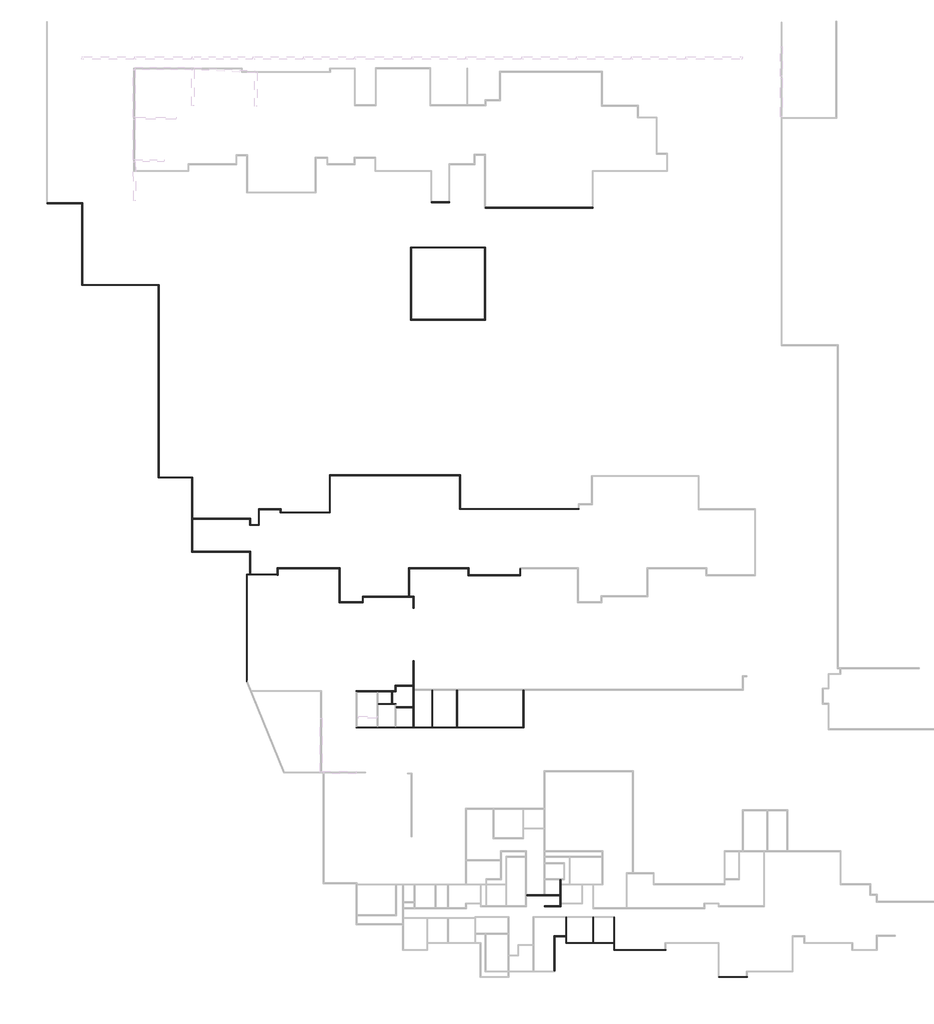
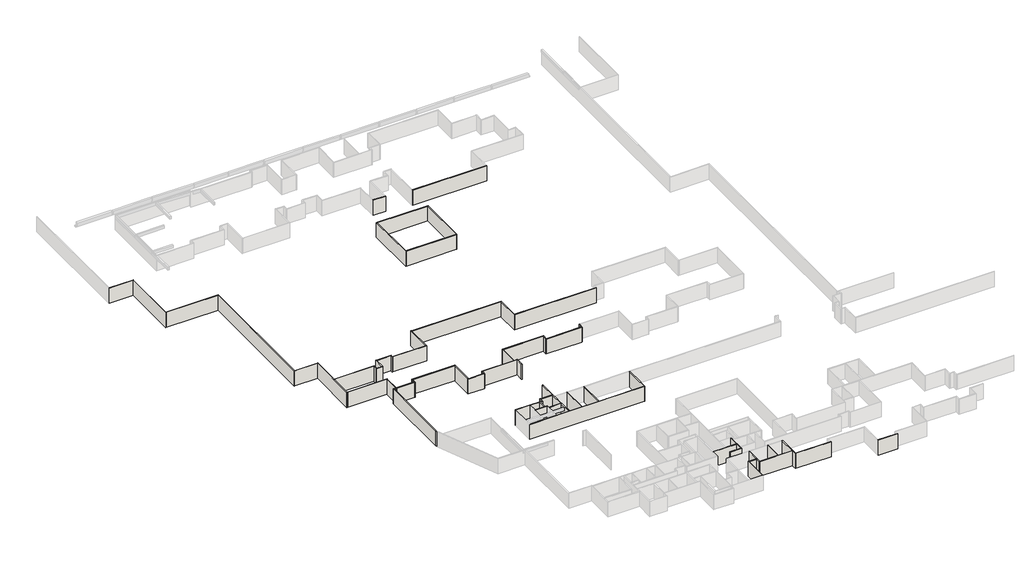
# One storey, part 2 of 8: 63 walls.
"""IFC4 building model written with IfcOpenShell, lengths in millimetres."""

from ifc_helpers import new_model, si_unit, origin, origin_with_axes, place, context, project, spatial, polyline, outline, extrude, faceted_brep, element, save

model = new_model("IFC4")

# Units and contexts
model_context = context("Model", 3, world=origin())
ifc_project = project(units=[si_unit("LENGTHUNIT", "METRE", prefix="MILLI")], contexts=[model_context])

# Site, building, storey
site = spatial("IfcSite", under=ifc_project)
building = spatial("IfcBuilding", under=site)
storey = spatial("IfcBuildingStorey", under=building, Name="户型图", Elevation=0.0)

# Walls
placement = place(None, origin())
element("IfcWall", 1, ObjectType="所有墙体", at=placement, inside=storey, context=model_context, shape_type="Brep", body=[
    faceted_brep([(57170.338145, 126907.0451941, 0.0), (62113.8430954, 126907.0451941, 0.0), (62113.8430954, 126907.0451941, 3300.0), (57170.338145, 126907.0451941, 3300.0), (57170.338145, 127027.0451941, 0.0), (57170.338145, 127027.0451941, 3300.0), (62108.8476291, 127027.0451941, 3300.0), (62113.8430954, 127027.0451941, 3300.0), (62113.8430954, 127027.0451941, 0.0)], [[[0, 1, 2, 3]], [[4, 5, 6, 7, 8]], [[1, 0, 4, 8]], [[3, 2, 7, 6, 5]], [[2, 1, 8, 7]], [[0, 3, 5, 4]]]),
])
element("IfcWall", 2, ObjectType="所有墙体", at=placement, inside=storey, context=model_context, shape_type="Brep", body=[
    faceted_brep([(62113.8430954, 127027.0451941, 0.0), (62113.8430954, 126907.0451941, 0.0), (62113.8430954, 115127.0451941, 0.0), (62113.8430954, 115127.0451941, 3300.0), (62113.8430954, 126907.0451941, 3300.0), (62113.8430954, 127027.0451941, 3300.0), (62233.8430954, 127027.0451941, 0.0), (62233.8430954, 127027.0451941, 2700.0), (62233.8430954, 127027.0451941, 3300.0), (62233.8430954, 126967.1449171, 3300.0), (62233.8430954, 115247.0451941, 3300.0), (62233.8430954, 115127.0451941, 3300.0), (62233.8430954, 115127.0451941, 0.0), (62233.8430954, 115247.0451941, 0.0)], [[[0, 1, 2, 3, 4, 5]], [[6, 7, 8, 9, 10, 11, 12, 13]], [[2, 1, 0, 6, 13, 12]], [[5, 4, 3, 11, 10, 9, 8]], [[0, 5, 8, 7, 6]], [[3, 2, 12, 11]]]),
])
element("IfcWall", 3, ObjectType="所有墙体", at=placement, inside=storey, context=model_context, shape_type="Brep", body=[
    faceted_brep([(62233.8430954, 115127.0451941, 0.0), (73113.8430954, 115127.0451941, 0.0), (73233.8430954, 115127.0451941, 0.0), (73233.8430954, 115127.0451941, 3300.0), (73113.8430954, 115127.0451941, 3300.0), (62233.8430954, 115127.0451941, 3300.0), (62233.8430954, 115247.0451941, 0.0), (62233.8430954, 115247.0451941, 3300.0), (73233.8430954, 115247.0451941, 3300.0), (73233.8430954, 115247.0451941, 0.0)], [[[0, 1, 2, 3, 4, 5]], [[6, 7, 8, 9]], [[2, 1, 0, 6, 9]], [[5, 4, 3, 8, 7]], [[0, 5, 7, 6]], [[3, 2, 9, 8]]]),
])
element("IfcWall", 4, ObjectType="所有墙体", at=placement, inside=storey, context=model_context, shape_type="Brep", body=[
    faceted_brep([(73113.8430954, 115127.0451941, 0.0), (73113.8430954, 87427.0451941, 0.0), (73113.8430954, 87427.0451941, 3300.0), (73113.8430954, 115127.0451941, 3300.0), (73233.8430954, 115127.0451941, 0.0), (73233.8430954, 115127.0451941, 3300.0), (73233.8430954, 87547.0451941, 3300.0), (73233.8430954, 87427.0451941, 3300.0), (73233.8430954, 87427.0451941, 0.0), (73233.8430954, 87547.0451941, 0.0)], [[[0, 1, 2, 3]], [[4, 5, 6, 7, 8, 9]], [[1, 0, 4, 9, 8]], [[3, 2, 7, 6, 5]], [[0, 3, 5, 4]], [[2, 1, 8, 7]]]),
])
element("IfcWall", 5, ObjectType="所有墙体", at=placement, inside=storey, context=model_context, shape_type="Brep", body=[
    faceted_brep([(73233.8430954, 87427.0451941, 0.0), (77963.8475536, 87427.0451941, 0.0), (78083.8475536, 87427.0451941, 0.0), (78083.8475536, 87427.0451941, 3300.0), (77963.8475536, 87427.0451941, 3300.0), (73233.8430954, 87427.0451941, 3300.0), (73233.8430954, 87547.0451941, 0.0), (73233.8430954, 87547.0451941, 3300.0), (77970.8225114, 87547.0451941, 3300.0), (78083.8475536, 87547.0451941, 3300.0), (78083.8475536, 87547.0451941, 2700.0), (78083.8475536, 87547.0451941, 0.0)], [[[0, 1, 2, 3, 4, 5]], [[6, 7, 8, 9, 10, 11]], [[2, 1, 0, 6, 11]], [[5, 4, 3, 9, 8, 7]], [[0, 5, 7, 6]], [[3, 2, 11, 10, 9]]]),
])
element("IfcWall", 6, ObjectType="所有墙体", at=placement, inside=storey, context=model_context, shape_type="Brep", body=[
    faceted_brep([(77963.8475536, 87427.0451941, 0.0), (77963.8475536, 76756.9488348, 0.0), (77963.8475536, 76756.9488348, 3300.0), (77963.8475536, 87427.0451941, 3300.0), (78083.8475536, 87427.0451941, 0.0), (78083.8475536, 87427.0451941, 3300.0), (78083.8475536, 87285.4298587, 3300.0), (78083.8475536, 87274.6689745, 3300.0), (78083.8475536, 76876.9488348, 3300.0), (78083.8475536, 76756.9488348, 3300.0), (78083.8475536, 76756.9488348, 0.0), (78083.8475536, 76876.9488348, 0.0)], [[[0, 1, 2, 3]], [[4, 5, 6, 7, 8, 9, 10, 11]], [[1, 0, 4, 11, 10]], [[3, 2, 9, 8, 7, 6, 5]], [[0, 3, 5, 4]], [[2, 1, 10, 9]]]),
])
element("IfcWall", 7, ObjectType="所有墙体", at=placement, inside=storey, context=model_context, shape_type="Brep", body=[
    faceted_brep([(78083.8475536, 76756.9488348, 0.0), (86321.4607933, 76756.9488348, 0.0), (86441.4607933, 76756.9488348, 0.0), (86441.4607933, 76756.9488348, 3300.0), (86321.4607933, 76756.9488348, 3300.0), (78083.8475536, 76756.9488348, 3300.0), (78083.8475536, 76876.9488348, 0.0), (78083.8475536, 76876.9488348, 3300.0), (86441.4607933, 76876.9488348, 3300.0), (86441.4607933, 76876.9488348, 0.0)], [[[0, 1, 2, 3, 4, 5]], [[6, 7, 8, 9]], [[2, 1, 0, 6, 9]], [[5, 4, 3, 8, 7]], [[0, 5, 7, 6]], [[3, 2, 9, 8]]]),
])
element("IfcWall", 8, ObjectType="所有墙体", at=placement, inside=storey, context=model_context, shape_type="Brep", body=[
    faceted_brep([(86321.4607933, 76756.9488348, 0.0), (86321.4607933, 73602.0351588, 0.0), (86321.4607933, 73482.0351588, 0.0), (86321.4607933, 73482.0351588, 3300.0), (86321.4607933, 73602.0351588, 3300.0), (86321.4607933, 76756.9488348, 3300.0), (86441.4607933, 76756.9488348, 0.0), (86441.4607933, 76756.9488348, 3300.0), (86441.4607933, 73482.0351588, 3300.0), (86441.4607933, 73482.0351588, 0.0)], [[[0, 1, 2, 3, 4, 5]], [[6, 7, 8, 9]], [[2, 1, 0, 6, 9]], [[5, 4, 3, 8, 7]], [[0, 5, 7, 6]], [[3, 2, 9, 8]]]),
])
element("IfcWall", 9, ObjectType="所有墙体", at=placement, inside=storey, context=model_context, shape_type="Brep", body=[
    faceted_brep([(86321.4607933, 73602.0351588, 0.0), (85838.8477345, 73602.0351588, 0.0), (85838.8477345, 73602.0351588, 3300.0), (86321.4607933, 73602.0351588, 3300.0), (86321.4607933, 73482.0351588, 0.0), (86321.4607933, 73482.0351588, 3300.0), (85958.8477345, 73482.0351588, 3300.0), (85838.8477345, 73482.0351588, 3300.0), (85838.8477345, 73482.0351588, 0.0), (85958.8477345, 73482.0351588, 0.0)], [[[0, 1, 2, 3]], [[4, 5, 6, 7, 8, 9]], [[1, 0, 4, 9, 8]], [[3, 2, 7, 6, 5]], [[0, 3, 5, 4]], [[2, 1, 8, 7]]]),
])
element("IfcWall", 10, ObjectType="所有墙体", at=placement, inside=storey, context=model_context, shape_type="Brep", body=[
    faceted_brep([(85838.8477345, 73482.0351588, 0.0), (85838.8477345, 58187.0147251, 0.0), (85838.8477345, 58187.0147251, 3300.0), (85838.8477345, 73482.0351588, 3300.0), (85958.8477345, 73482.0351588, 0.0), (85958.8477345, 73482.0351588, 3300.0), (85958.8477345, 58210.3403622, 3300.0), (85958.8477345, 57890.0043027, 3300.0), (85958.8477345, 57890.0043027, 0.0), (85958.8477345, 58210.3403622, 0.0)], [[[0, 1, 2, 3]], [[4, 5, 6, 7, 8, 9]], [[1, 0, 4, 9, 8]], [[3, 2, 7, 6, 5]], [[0, 3, 5, 4]], [[2, 1, 8, 7]]]),
])
element("IfcWall", 11, ObjectType="所有墙体", at=placement, inside=storey, context=model_context, shape_type="SweptSolid", body=[
    extrude(outline(polyline([(130227.9809927, 21540.9349261), (130227.9809927, 16465.6854162), (130107.9809927, 16465.6854162), (130107.9809927, 21540.9349261), (130227.9809927, 21540.9349261)])), origin_with_axes(), (0.0, 0.0, 1.0), 3300.0),
])
element("IfcWall", 12, ObjectType="所有墙体", at=placement, inside=storey, context=model_context, shape_type="SweptSolid", body=[
    extrude(outline(polyline([(131807.9809889, 21420.9349261), (130227.9809927, 21420.9349261), (130227.9809927, 21540.9349261), (131807.9809889, 21540.9349261), (131807.9809889, 21420.9349261)])), origin_with_axes(), (0.0, 0.0, 1.0), 3300.0),
])
element("IfcWall", 13, ObjectType="所有墙体", at=placement, inside=storey, context=model_context, shape_type="Brep", body=[
    faceted_brep([(131807.9809889, 24196.1844453, 0.0), (131807.9809889, 21540.9349261, 0.0), (131807.9809889, 21420.9349261, 0.0), (131807.9809889, 20445.6854108, 0.0), (131807.9809889, 20445.6854108, 3300.0), (131807.9809889, 21420.9349261, 3300.0), (131807.9809889, 21540.9349261, 3300.0), (131807.9809889, 24196.1844453, 3300.0), (131927.9809889, 24196.1844453, 0.0), (131927.9809889, 24196.1844453, 3300.0), (131927.9809889, 20565.6854108, 3300.0), (131927.9809889, 20445.6854108, 3300.0), (131927.9809889, 20445.6854108, 0.0), (131927.9809889, 20565.6854108, 0.0)], [[[0, 1, 2, 3, 4, 5, 6, 7]], [[8, 9, 10, 11, 12, 13]], [[3, 2, 1, 0, 8, 13, 12]], [[7, 6, 5, 4, 11, 10, 9]], [[4, 3, 12, 11]], [[0, 7, 9, 8]]]),
])
element("IfcWall", 14, ObjectType="所有墙体", at=placement, inside=storey, context=model_context, shape_type="Brep", body=[
    faceted_brep([(131927.9809889, 20445.6854108, 0.0), (138707.9809942, 20445.6854108, 0.0), (138707.9809942, 20445.6854108, 3300.0), (131927.9809889, 20445.6854108, 3300.0), (131927.9809889, 20565.6854108, 0.0), (131927.9809889, 20565.6854108, 3300.0), (135707.98099, 20565.6854108, 3300.0), (135827.98099, 20565.6854108, 3300.0), (138707.9809941, 20565.6854108, 3300.0), (138707.9809941, 20565.6854108, 0.0), (135827.98099, 20565.6854108, 0.0), (135707.98099, 20565.6854108, 0.0)], [[[0, 1, 2, 3]], [[4, 5, 6, 7, 8, 9, 10, 11]], [[1, 0, 4, 11, 10, 9]], [[3, 2, 8, 7, 6, 5]], [[0, 3, 5, 4]], [[2, 1, 9, 8]]]),
])
element("IfcWall", 15, ObjectType="所有墙体", at=placement, inside=storey, context=model_context, shape_type="Brep", body=[
    faceted_brep([(138707.9809916, 24196.1844453, 0.0), (138707.9809941, 20565.6854108, 0.0), (138707.9809942, 20445.6854108, 0.0), (138707.9809949, 19445.6854079, 0.0), (138707.9809949, 19445.6854079, 3300.0), (138707.9809942, 20445.6854108, 3300.0), (138707.9809941, 20565.6854108, 3300.0), (138707.9809916, 24196.1844453, 3300.0), (138827.9809916, 24196.1844453, 0.0), (138827.9809916, 24196.1844453, 3300.0), (138827.9809949, 19445.6854079, 3300.0), (138827.9809949, 19445.6854079, 0.0)], [[[0, 1, 2, 3, 4, 5, 6, 7]], [[8, 9, 10, 11]], [[3, 2, 1, 0, 8, 11]], [[7, 6, 5, 4, 10, 9]], [[4, 3, 11, 10]], [[0, 7, 9, 8]]]),
])
element("IfcWall", 16, ObjectType="所有墙体", at=placement, inside=storey, context=model_context, shape_type="Brep", body=[
    faceted_brep([(138827.9809949, 19445.6854079, 0.0), (146227.9809999, 19445.6854079, 0.0), (146227.9809999, 19445.6854079, 3300.0), (138827.9809949, 19445.6854079, 3300.0), (138827.9809949, 19565.6854079, 0.0), (138827.9809949, 19565.6854079, 3300.0), (146107.9809999, 19565.6854079, 3300.0), (146227.9809999, 19565.6854079, 3300.0), (146227.9809999, 19565.6854079, 0.0), (146107.9809999, 19565.6854079, 0.0)], [[[0, 1, 2, 3]], [[4, 5, 6, 7, 8, 9]], [[1, 0, 4, 9, 8]], [[3, 2, 7, 6, 5]], [[0, 3, 5, 4]], [[2, 1, 8, 7]]]),
])
element("IfcWall", 17, ObjectType="所有墙体", at=placement, inside=storey, context=model_context, shape_type="Brep", body=[
    faceted_brep([(153877.9809859, 15545.6854108, 0.0), (157927.981003, 15545.6854108, 0.0), (157927.981003, 15545.6854108, 3300.0), (153877.9809859, 15545.6854108, 3300.0), (153877.9809859, 15665.6854108, 0.0), (153877.9809859, 15665.6854108, 3300.0), (157807.981003, 15665.6854108, 3300.0), (157927.981003, 15665.6854108, 3300.0), (157927.981003, 15665.6854108, 0.0), (157807.981003, 15665.6854108, 0.0)], [[[0, 1, 2, 3]], [[4, 5, 6, 7, 8, 9]], [[1, 0, 4, 9, 8]], [[3, 2, 7, 6, 5]], [[0, 3, 5, 4]], [[2, 1, 8, 7]]]),
])
element("IfcWall", 18, ObjectType="所有墙体", at=placement, inside=storey, context=model_context, shape_type="Brep", body=[
    faceted_brep([(112508.8239737, 127056.6496336, 0.0), (115083.8238911, 127056.6496336, 0.0), (115083.8238911, 127056.6496336, 3300.0), (112508.8239737, 127056.6496336, 3300.0), (112508.8239737, 127176.6496336, 0.0), (112508.8239737, 127176.6496336, 3300.0), (114963.8238911, 127176.6496336, 3300.0), (115083.8238911, 127176.6496336, 3300.0), (115083.8238911, 127176.6496336, 0.0), (114963.8238911, 127176.6496336, 0.0)], [[[0, 1, 2, 3]], [[4, 5, 6, 7, 8, 9]], [[1, 0, 4, 9, 8]], [[3, 2, 7, 6, 5]], [[0, 3, 5, 4]], [[2, 1, 8, 7]]]),
])
element("IfcWall", 19, ObjectType="所有墙体", at=placement, inside=storey, context=model_context, shape_type="Brep", body=[
    faceted_brep([(120252.3761316, 126236.2446076, 0.0), (135753.7737349, 126236.2446076, 0.0), (135753.7737349, 126236.2446076, 3300.0), (120252.3761316, 126236.2446076, 3300.0), (120252.3761316, 126356.2446076, 0.0), (120252.3761316, 126356.2446076, 3300.0), (135633.7737349, 126356.2446076, 3300.0), (135753.7737349, 126356.2446076, 3300.0), (135753.7737349, 126356.2446076, 0.0), (135633.7737349, 126356.2446076, 0.0)], [[[0, 1, 2, 3]], [[4, 5, 6, 7, 8, 9]], [[1, 0, 4, 9, 8]], [[3, 2, 7, 6, 5]], [[0, 3, 5, 4]], [[2, 1, 8, 7]]]),
])
element("IfcWall", 20, ObjectType="所有墙体", at=placement, inside=storey, context=model_context, shape_type="Brep", body=[
    faceted_brep([(78083.8475536, 81506.8474053, 0.0), (86321.4607933, 81506.8474053, 0.0), (86441.4607933, 81506.8474053, 0.0), (86441.4607933, 81506.8474053, 3300.0), (86321.4607933, 81506.8474053, 3300.0), (78083.8475536, 81506.8474053, 3300.0), (78083.8475536, 81626.8474053, 0.0), (78083.8475536, 81626.8474053, 3300.0), (86441.4607933, 81626.8474053, 3300.0), (86441.4607933, 81626.8474053, 0.0)], [[[0, 1, 2, 3, 4, 5]], [[6, 7, 8, 9]], [[2, 1, 0, 6, 9]], [[5, 4, 3, 8, 7]], [[0, 5, 7, 6]], [[3, 2, 9, 8]]]),
])
element("IfcWall", 21, ObjectType="所有墙体", at=placement, inside=storey, context=model_context, shape_type="Brep", body=[
    faceted_brep([(86321.4607933, 81506.8474053, 0.0), (86321.4607933, 80582.2150761, 0.0), (86321.4607933, 80582.2150761, 3300.0), (86321.4607933, 81506.8474053, 3300.0), (86441.4607933, 81506.8474053, 0.0), (86441.4607933, 81506.8474053, 3300.0), (86441.4607933, 80702.2150761, 3300.0), (86441.4607933, 80582.2150761, 3300.0), (86441.4607933, 80582.2150761, 0.0), (86441.4607933, 80702.2150761, 0.0)], [[[0, 1, 2, 3]], [[4, 5, 6, 7, 8, 9]], [[1, 0, 4, 9, 8]], [[3, 2, 7, 6, 5]], [[0, 3, 5, 4]], [[2, 1, 8, 7]]]),
])
element("IfcWall", 22, ObjectType="所有墙体", at=placement, inside=storey, context=model_context, shape_type="Brep", body=[
    faceted_brep([(86441.4607933, 80582.2150761, 0.0), (87690.2437459, 80582.2150761, 0.0), (87690.2437459, 80582.2150761, 3300.0), (86441.4607933, 80582.2150761, 3300.0), (86441.4607933, 80702.2150761, 0.0), (86441.4607933, 80702.2150761, 3300.0), (87570.2437459, 80702.2150761, 3300.0), (87690.2437459, 80702.2150761, 3300.0), (87690.2437459, 80702.2150761, 0.0), (87570.2437459, 80702.2150761, 0.0)], [[[0, 1, 2, 3]], [[4, 5, 6, 7, 8, 9]], [[1, 0, 4, 9, 8]], [[3, 2, 7, 6, 5]], [[0, 3, 5, 4]], [[2, 1, 8, 7]]]),
])
element("IfcWall", 23, ObjectType="所有墙体", at=placement, inside=storey, context=model_context, shape_type="Brep", body=[
    faceted_brep([(87690.2437459, 80702.2150761, 0.0), (87690.2437459, 82883.5885663, 0.0), (87690.2437459, 83003.5885663, 0.0), (87690.2437459, 83003.5885663, 3300.0), (87690.2437459, 82883.5885663, 3300.0), (87690.2437459, 80702.2150761, 3300.0), (87570.2437459, 80702.2150761, 0.0), (87570.2437459, 80702.2150761, 3300.0), (87570.2437459, 83003.5885663, 3300.0), (87570.2437459, 83003.5885663, 0.0)], [[[0, 1, 2, 3, 4, 5]], [[6, 7, 8, 9]], [[2, 1, 0, 6, 9]], [[5, 4, 3, 8, 7]], [[0, 5, 7, 6]], [[3, 2, 9, 8]]]),
])
element("IfcWall", 24, ObjectType="所有墙体", at=placement, inside=storey, context=model_context, shape_type="Brep", body=[
    faceted_brep([(87690.2437459, 82883.5885663, 0.0), (90670.6043252, 82883.5885663, 0.0), (90790.6043252, 82883.5885663, 0.0), (90790.6043252, 82883.5885663, 3300.0), (90670.6043252, 82883.5885663, 3300.0), (87690.2437459, 82883.5885663, 3300.0), (87690.2437459, 83003.5885663, 0.0), (87690.2437459, 83003.5885663, 3300.0), (90790.6043252, 83003.5885663, 3300.0), (90790.6043252, 83003.5885663, 0.0)], [[[0, 1, 2, 3, 4, 5]], [[6, 7, 8, 9]], [[2, 1, 0, 6, 9]], [[5, 4, 3, 8, 7]], [[0, 5, 7, 6]], [[3, 2, 9, 8]]]),
])
element("IfcWall", 25, ObjectType="所有墙体", at=placement, inside=storey, context=model_context, shape_type="Brep", body=[
    faceted_brep([(90670.6043252, 82883.5885663, 0.0), (90670.6043252, 82384.1590771, 0.0), (90670.6043252, 82384.1590771, 3300.0), (90670.6043252, 82883.5885663, 3300.0), (90790.6043252, 82883.5885663, 0.0), (90790.6043252, 82883.5885663, 3300.0), (90790.6043252, 82504.1590771, 3300.0), (90790.6043252, 82384.1590771, 3300.0), (90790.6043252, 82384.1590771, 0.0), (90790.6043252, 82504.1590771, 0.0)], [[[0, 1, 2, 3]], [[4, 5, 6, 7, 8, 9]], [[1, 0, 4, 9, 8]], [[3, 2, 7, 6, 5]], [[0, 3, 5, 4]], [[2, 1, 8, 7]]]),
])
element("IfcWall", 26, ObjectType="所有墙体", at=placement, inside=storey, context=model_context, shape_type="Brep", body=[
    faceted_brep([(90790.6043252, 82384.1590771, 0.0), (97890.3252987, 82384.1590771, 0.0), (97890.3252987, 82384.1590771, 3300.0), (90790.6043252, 82384.1590771, 3300.0), (90790.6043252, 82504.1590771, 0.0), (90790.6043252, 82504.1590771, 3300.0), (97770.3252987, 82504.1590771, 3300.0), (97890.3252987, 82504.1590771, 3300.0), (97890.3252987, 82504.1590771, 0.0), (97770.3252987, 82504.1590771, 0.0)], [[[0, 1, 2, 3]], [[4, 5, 6, 7, 8, 9]], [[1, 0, 4, 9, 8]], [[3, 2, 7, 6, 5]], [[0, 3, 5, 4]], [[2, 1, 8, 7]]]),
])
element("IfcWall", 27, ObjectType="所有墙体", at=placement, inside=storey, context=model_context, shape_type="Brep", body=[
    faceted_brep([(97890.3252987, 82504.1590771, 0.0), (97890.3252987, 87734.182849, 0.0), (97890.3252987, 87854.182849, 0.0), (97890.3252987, 87854.182849, 3300.0), (97890.3252987, 87734.182849, 3300.0), (97890.3252987, 82504.1590771, 3300.0), (97770.3252987, 82504.1590771, 0.0), (97770.3252987, 82504.1590771, 3300.0), (97770.3252987, 87854.182849, 3300.0), (97770.3252987, 87854.182849, 0.0)], [[[0, 1, 2, 3, 4, 5]], [[6, 7, 8, 9]], [[2, 1, 0, 6, 9]], [[5, 4, 3, 8, 7]], [[0, 5, 7, 6]], [[3, 2, 9, 8]]]),
])
element("IfcWall", 28, ObjectType="所有墙体", at=placement, inside=storey, context=model_context, shape_type="Brep", body=[
    faceted_brep([(97890.3252987, 87734.182849, 0.0), (116520.1629656, 87734.182849, 0.0), (116640.1629656, 87734.182849, 0.0), (116640.1629656, 87734.182849, 3300.0), (116520.1629656, 87734.182849, 3300.0), (97890.3252987, 87734.182849, 3300.0), (97890.3252987, 87854.182849, 0.0), (97890.3252987, 87854.182849, 3300.0), (116640.1629656, 87854.182849, 3300.0), (116640.1629656, 87854.182849, 0.0)], [[[0, 1, 2, 3, 4, 5]], [[6, 7, 8, 9]], [[2, 1, 0, 6, 9]], [[5, 4, 3, 8, 7]], [[0, 5, 7, 6]], [[3, 2, 9, 8]]]),
])
element("IfcWall", 29, ObjectType="所有墙体", at=placement, inside=storey, context=model_context, shape_type="Brep", body=[
    faceted_brep([(116520.1629656, 87734.182849, 0.0), (116520.1629656, 82888.343556, 0.0), (116520.1629656, 82888.343556, 3300.0), (116520.1629656, 87734.182849, 3300.0), (116640.1629656, 87734.182849, 0.0), (116640.1629656, 87734.182849, 3300.0), (116640.1629656, 83008.343556, 3300.0), (116640.1629656, 82888.343556, 3300.0), (116640.1629656, 82888.343556, 0.0), (116640.1629656, 83008.343556, 0.0)], [[[0, 1, 2, 3]], [[4, 5, 6, 7, 8, 9]], [[1, 0, 4, 9, 8]], [[3, 2, 7, 6, 5]], [[0, 3, 5, 4]], [[2, 1, 8, 7]]]),
])
element("IfcWall", 30, ObjectType="所有墙体", at=placement, inside=storey, context=model_context, shape_type="Brep", body=[
    faceted_brep([(116640.1629656, 82888.343556, 0.0), (133740.1629656, 82888.343556, 0.0), (133740.1629656, 82888.343556, 3300.0), (116640.1629656, 82888.343556, 3300.0), (116640.1629656, 83008.343556, 0.0), (116640.1629656, 83008.343556, 3300.0), (133620.1629656, 83008.343556, 3300.0), (133740.1629656, 83008.343556, 3300.0), (133740.1629656, 83008.343556, 0.0), (133620.1629656, 83008.343556, 0.0)], [[[0, 1, 2, 3]], [[4, 5, 6, 7, 8, 9]], [[1, 0, 4, 9, 8]], [[3, 2, 7, 6, 5]], [[0, 3, 5, 4]], [[2, 1, 8, 7]]]),
])
element("IfcWall", 31, ObjectType="所有墙体", at=placement, inside=storey, context=model_context, shape_type="Brep", body=[
    faceted_brep([(125182.2319998, 74387.635971, 0.0), (125182.2319998, 73504.4568159, 0.0), (125182.2319998, 73384.4568159, 0.0), (125182.2319998, 73384.4568159, 3300.0), (125182.2319998, 73504.4568159, 3300.0), (125182.2319998, 74387.635971, 3300.0), (125302.2319998, 74387.635971, 0.0), (125302.2319998, 74387.635971, 3300.0), (125302.2319998, 73384.4568159, 3300.0), (125302.2319998, 73384.4568159, 0.0)], [[[0, 1, 2, 3, 4, 5]], [[6, 7, 8, 9]], [[2, 1, 0, 6, 9]], [[5, 4, 3, 8, 7]], [[0, 5, 7, 6]], [[3, 2, 9, 8]]]),
])
element("IfcWall", 32, ObjectType="所有墙体", at=placement, inside=storey, context=model_context, shape_type="Brep", body=[
    faceted_brep([(125182.2319998, 73504.4568159, 0.0), (117841.6020426, 73504.4568159, 0.0), (117721.6020426, 73504.4568159, 0.0), (117721.6020426, 73504.4568159, 3300.0), (117841.6020426, 73504.4568159, 3300.0), (125182.2319998, 73504.4568159, 3300.0), (125182.2319998, 73384.4568159, 0.0), (125182.2319998, 73384.4568159, 3300.0), (117721.6020426, 73384.4568159, 3300.0), (117721.6020426, 73384.4568159, 0.0)], [[[0, 1, 2, 3, 4, 5]], [[6, 7, 8, 9]], [[2, 1, 0, 6, 9]], [[5, 4, 3, 8, 7]], [[0, 5, 7, 6]], [[3, 2, 9, 8]]]),
])
element("IfcWall", 33, ObjectType="所有墙体", at=placement, inside=storey, context=model_context, shape_type="Brep", body=[
    faceted_brep([(117841.6020426, 73504.4568159, 0.0), (117841.6020426, 74507.635971, 0.0), (117841.6020426, 74507.635971, 3300.0), (117841.6020426, 73504.4568159, 3300.0), (117721.6020426, 73504.4568159, 0.0), (117721.6020426, 73504.4568159, 3300.0), (117721.6020426, 74387.635971, 3300.0), (117721.6020426, 74507.635971, 3300.0), (117721.6020426, 74507.635971, 0.0), (117721.6020426, 74387.635971, 0.0)], [[[0, 1, 2, 3]], [[4, 5, 6, 7, 8, 9]], [[1, 0, 4, 9, 8]], [[3, 2, 7, 6, 5]], [[0, 3, 5, 4]], [[2, 1, 8, 7]]]),
])
element("IfcWall", 34, ObjectType="所有墙体", at=placement, inside=storey, context=model_context, shape_type="Brep", body=[
    faceted_brep([(117721.6020426, 74507.635971, 0.0), (109172.5505836, 74507.635971, 0.0), (109172.5505836, 74507.635971, 3300.0), (117721.6020426, 74507.635971, 3300.0), (117721.6020426, 74387.635971, 0.0), (117721.6020426, 74387.635971, 3300.0), (109292.5505836, 74387.635971, 3300.0), (109172.5505836, 74387.635971, 3300.0), (109172.5505836, 74387.635971, 0.0), (109292.5505836, 74387.635971, 0.0)], [[[0, 1, 2, 3]], [[4, 5, 6, 7, 8, 9]], [[1, 0, 4, 9, 8]], [[3, 2, 7, 6, 5]], [[0, 3, 5, 4]], [[2, 1, 8, 7]]]),
])
element("IfcWall", 35, ObjectType="所有墙体", at=placement, inside=storey, context=model_context, shape_type="SweptSolid", body=[
    extrude(outline(polyline([(109172.5505836, 70405.0152295), (109172.5505836, 74387.635971), (109292.5505836, 74387.635971), (109292.5505836, 70405.0152295), (109172.5505836, 70405.0152295)])), origin_with_axes(), (0.0, 0.0, 1.0), 3300.0),
])
element("IfcWall", 36, ObjectType="所有墙体", at=placement, inside=storey, context=model_context, shape_type="Brep", body=[
    faceted_brep([(109958.7128377, 70405.0152295, 0.0), (109292.5505836, 70405.0152295, 0.0), (109172.5505836, 70405.0152295, 0.0), (102523.1323386, 70405.0152295, 0.0), (102523.1323386, 70405.0152295, 3300.0), (109172.5505836, 70405.0152295, 3300.0), (109292.5505836, 70405.0152295, 3300.0), (109958.7128377, 70405.0152295, 3300.0), (109958.7128377, 70285.0152295, 0.0), (109958.7128377, 70285.0152295, 3300.0), (109838.7128377, 70285.0152295, 3300.0), (102643.1323386, 70285.0152295, 3300.0), (102523.1323386, 70285.0152295, 3300.0), (102523.1323386, 70285.0152295, 0.0), (102643.1323386, 70285.0152295, 0.0), (109838.7128377, 70285.0152295, 0.0)], [[[0, 1, 2, 3, 4, 5, 6, 7]], [[8, 9, 10, 11, 12, 13, 14, 15]], [[3, 2, 1, 0, 8, 15, 14, 13]], [[7, 6, 5, 4, 12, 11, 10, 9]], [[4, 3, 13, 12]], [[0, 7, 9, 8]]]),
])
element("IfcWall", 37, ObjectType="所有墙体", at=placement, inside=storey, context=model_context, shape_type="Brep", body=[
    faceted_brep([(102523.1323386, 70285.0152295, 0.0), (102523.1323386, 69603.7624578, 0.0), (102523.1323386, 69483.7624578, 0.0), (102523.1323386, 69483.7624578, 3300.0), (102523.1323386, 69603.7624578, 3300.0), (102523.1323386, 70285.0152295, 3300.0), (102643.1323386, 70285.0152295, 0.0), (102643.1323386, 70285.0152295, 3300.0), (102643.1323386, 69483.7624578, 3300.0), (102643.1323386, 69483.7624578, 0.0)], [[[0, 1, 2, 3, 4, 5]], [[6, 7, 8, 9]], [[2, 1, 0, 6, 9]], [[5, 4, 3, 8, 7]], [[0, 5, 7, 6]], [[3, 2, 9, 8]]]),
])
element("IfcWall", 38, ObjectType="所有墙体", at=placement, inside=storey, context=model_context, shape_type="Brep", body=[
    faceted_brep([(102523.1323386, 69603.7624578, 0.0), (99291.7788422, 69603.7624578, 0.0), (99171.7788422, 69603.7624578, 0.0), (99171.7788422, 69603.7624578, 3300.0), (99291.7788422, 69603.7624578, 3300.0), (102523.1323386, 69603.7624578, 3300.0), (102523.1323386, 69483.7624578, 0.0), (102523.1323386, 69483.7624578, 3300.0), (99171.7788422, 69483.7624578, 3300.0), (99171.7788422, 69483.7624578, 0.0)], [[[0, 1, 2, 3, 4, 5]], [[6, 7, 8, 9]], [[2, 1, 0, 6, 9]], [[5, 4, 3, 8, 7]], [[0, 5, 7, 6]], [[3, 2, 9, 8]]]),
])
element("IfcWall", 39, ObjectType="所有墙体", at=placement, inside=storey, context=model_context, shape_type="Brep", body=[
    faceted_brep([(99291.7788422, 69603.7624578, 0.0), (99291.7788422, 74503.7624578, 0.0), (99291.7788422, 74503.7624578, 3300.0), (99291.7788422, 69603.7624578, 3300.0), (99171.7788422, 69603.7624578, 0.0), (99171.7788422, 69603.7624578, 3300.0), (99171.7788422, 74383.7624578, 3300.0), (99171.7788422, 74503.7624578, 3300.0), (99171.7788422, 74503.7624578, 0.0), (99171.7788422, 74383.7624578, 0.0)], [[[0, 1, 2, 3]], [[4, 5, 6, 7, 8, 9]], [[1, 0, 4, 9, 8]], [[3, 2, 7, 6, 5]], [[0, 3, 5, 4]], [[2, 1, 8, 7]]]),
])
element("IfcWall", 40, ObjectType="所有墙体", at=placement, inside=storey, context=model_context, shape_type="Brep", body=[
    faceted_brep([(99171.7788422, 74503.7624578, 0.0), (90271.7788422, 74503.7624578, 0.0), (90271.7788422, 74503.7624578, 3300.0), (99171.7788422, 74503.7624578, 3300.0), (99171.7788422, 74383.7624578, 0.0), (99171.7788422, 74383.7624578, 3300.0), (90391.7788422, 74383.7624578, 3300.0), (90271.7788422, 74383.7624578, 3300.0), (90271.7788422, 74383.7624578, 0.0), (90391.7788422, 74383.7624578, 0.0)], [[[0, 1, 2, 3]], [[4, 5, 6, 7, 8, 9]], [[1, 0, 4, 9, 8]], [[3, 2, 7, 6, 5]], [[0, 3, 5, 4]], [[2, 1, 8, 7]]]),
])
element("IfcWall", 41, ObjectType="所有墙体", at=placement, inside=storey, context=model_context, shape_type="Brep", body=[
    faceted_brep([(90271.7788422, 74383.7624578, 0.0), (90271.7788422, 73602.0351588, 0.0), (90271.7788422, 73482.0351588, 0.0), (90271.7788422, 73442.0165642, 0.0), (90271.7788422, 73442.0165642, 3300.0), (90271.7788422, 73482.0351588, 3300.0), (90271.7788422, 73602.0351588, 3300.0), (90271.7788422, 74383.7624578, 3300.0), (90391.7788422, 74383.7624578, 0.0), (90391.7788422, 74383.7624578, 3300.0), (90391.7788422, 73442.0165642, 3300.0), (90391.7788422, 73442.0165642, 0.0)], [[[0, 1, 2, 3, 4, 5, 6, 7]], [[8, 9, 10, 11]], [[3, 2, 1, 0, 8, 11]], [[4, 3, 11, 10]], [[7, 6, 5, 4, 10, 9]], [[0, 7, 9, 8]]]),
])
element("IfcWall", 42, ObjectType="所有墙体", at=placement, inside=storey, context=model_context, shape_type="SweptSolid", body=[
    extrude(outline(polyline([(90271.7788422, 73482.0351588), (86441.4607933, 73482.0351588), (86441.4607933, 73602.0351588), (90271.7788422, 73602.0351588), (90271.7788422, 73482.0351588)])), origin_with_axes(), (0.0, 0.0, 1.0), 3300.0),
])
element("IfcWall", 43, ObjectType="所有墙体", at=placement, inside=storey, context=model_context, shape_type="Brep", body=[
    faceted_brep([(101638.8477337, 56681.8460485, 0.0), (101758.8477337, 56681.8460485, 0.0), (104655.6151291, 56681.8460485, 0.0), (104775.6151291, 56681.8460485, 0.0), (107358.8477337, 56681.8460485, 0.0), (107358.8477337, 56681.8460485, 3300.0), (104775.6151291, 56681.8460485, 3300.0), (104655.6151291, 56681.8460485, 3300.0), (101948.7128309, 56681.8460485, 3300.0), (101758.8477337, 56681.8460485, 3300.0), (101638.8477337, 56681.8460485, 3300.0), (101638.8477337, 56801.8460485, 0.0), (101638.8477337, 56801.8460485, 3300.0), (101648.7128309, 56801.8460485, 3300.0), (101948.7128309, 56801.8460485, 3300.0), (107238.8477337, 56801.8460485, 3300.0), (107358.8477337, 56801.8460485, 3300.0), (107358.8477337, 56801.8460485, 0.0), (107238.8477337, 56801.8460485, 0.0)], [[[0, 1, 2, 3, 4, 5, 6, 7, 8, 9, 10]], [[11, 12, 13, 14, 15, 16, 17, 18]], [[4, 3, 2, 1, 0, 11, 18, 17]], [[10, 9, 8, 7, 6, 5, 16, 15, 14, 13, 12]], [[5, 4, 17, 16]], [[0, 10, 12, 11]]]),
])
element("IfcWall", 44, ObjectType="所有墙体", at=placement, inside=storey, context=model_context, shape_type="Brep", body=[
    faceted_brep([(107358.8477337, 56801.8460485, 0.0), (107358.8477337, 57457.1438632, 0.0), (107358.8477337, 57577.1438632, 0.0), (107358.8477337, 57577.1438632, 3300.0), (107358.8477337, 57457.1438632, 3300.0), (107358.8477337, 56801.8460485, 3300.0), (107238.8477337, 56801.8460485, 0.0), (107238.8477337, 56801.8460485, 3300.0), (107238.8477337, 57577.1438632, 3300.0), (107238.8477337, 57577.1438632, 0.0)], [[[0, 1, 2, 3, 4, 5]], [[6, 7, 8, 9]], [[2, 1, 0, 6, 9]], [[5, 4, 3, 8, 7]], [[0, 5, 7, 6]], [[3, 2, 9, 8]]]),
])
element("IfcWall", 45, ObjectType="所有墙体", at=placement, inside=storey, context=model_context, shape_type="Brep", body=[
    faceted_brep([(107358.8477337, 57457.1438632, 0.0), (109838.7128377, 57457.1438632, 0.0), (109838.7128377, 57457.1438632, 2700.0), (109838.7128377, 57457.1438632, 3300.0), (109598.8477351, 57457.1438632, 3300.0), (107358.8477337, 57457.1438632, 3300.0), (107358.8477337, 57577.1438632, 0.0), (107358.8477337, 57577.1438632, 3300.0), (109598.8477351, 57577.1438632, 3300.0), (109838.7128377, 57577.1438632, 3300.0), (109838.7128377, 57577.1438632, 2700.0), (109838.7128377, 57577.1438632, 0.0)], [[[0, 1, 2, 3, 4, 5]], [[6, 7, 8, 9, 10, 11]], [[1, 0, 6, 11]], [[5, 4, 3, 9, 8, 7]], [[0, 5, 7, 6]], [[3, 2, 1, 11, 10, 9]]]),
])
element("IfcWall", 46, ObjectType="所有墙体", at=placement, inside=storey, context=model_context, shape_type="Brep", body=[
    faceted_brep([(109958.7128377, 54487.0649839, 0.0), (109958.7128377, 56907.0370398, 0.0), (109958.7128377, 57027.0370398, 0.0), (109958.7128377, 61154.2483952, 0.0), (109958.7128377, 61154.2483952, 3300.0), (109958.7128377, 61027.1438632, 3300.0), (109958.7128377, 60727.1438632, 3300.0), (109958.7128377, 57027.0370398, 3300.0), (109958.7128377, 56907.0370398, 3300.0), (109958.7128377, 54487.0649839, 3300.0), (109838.7128377, 54487.0649839, 0.0), (109838.7128377, 54487.0649839, 2700.0), (109838.7128377, 54487.0649839, 3300.0), (109838.7128377, 57457.1438632, 3300.0), (109838.7128377, 57577.1438632, 3300.0), (109838.7128377, 60727.1438632, 3300.0), (109838.7128377, 61027.1438632, 3300.0), (109838.7128377, 61154.2483952, 3300.0), (109838.7128377, 61154.2483952, 2700.0), (109838.7128377, 61154.2483952, 0.0), (109838.7128377, 57577.1438632, 0.0), (109838.7128377, 57457.1438632, 0.0), (109948.7128309, 61154.2483952, 3300.0)], [[[0, 1, 2, 3, 4, 5, 6, 7, 8, 9]], [[10, 11, 12, 13, 14, 15, 16, 17, 18, 19, 20, 21]], [[3, 2, 1, 0, 10, 21, 20, 19]], [[4, 3, 19, 18, 17, 22]], [[9, 8, 7, 6, 5, 4, 22, 17, 16, 15, 14, 13, 12]], [[0, 9, 12, 11, 10]]]),
])
element("IfcWall", 47, ObjectType="所有墙体", at=placement, inside=storey, context=model_context, shape_type="Brep", body=[
    faceted_brep([(125638.8240412, 56907.0370398, 0.0), (125638.8240412, 51576.8472247, 0.0), (125638.8240412, 51456.8472247, 0.0), (125638.8240412, 51456.8472247, 3300.0), (125638.8240412, 51576.8472247, 3300.0), (125638.8240412, 52782.6668088, 3300.0), (125638.8240412, 53082.6668088, 3300.0), (125638.8240412, 56907.0370398, 3300.0), (125638.8240412, 56907.0370398, 2700.0), (125758.8240412, 56907.0370398, 0.0), (125758.8240412, 56907.0370398, 2700.0), (125758.8240412, 56907.0370398, 3300.0), (125758.8240412, 53082.6668088, 3300.0), (125758.8240412, 52932.6668088, 3300.0), (125758.8240412, 51456.8472247, 3300.0), (125758.8240412, 51456.8472247, 2700.0), (125758.8240412, 51456.8472247, 0.0)], [[[0, 1, 2, 3, 4, 5, 6, 7, 8]], [[9, 10, 11, 12, 13, 14, 15, 16]], [[2, 1, 0, 9, 16]], [[7, 6, 5, 4, 3, 14, 13, 12, 11]], [[0, 8, 7, 11, 10, 9]], [[3, 2, 16, 15, 14]]]),
])
element("IfcWall", 48, ObjectType="所有墙体", at=placement, inside=storey, context=model_context, shape_type="Brep", body=[
    faceted_brep([(125638.8240412, 51576.8472247, 0.0), (107358.8477337, 51576.8472247, 0.0), (107238.8477337, 51576.8472247, 0.0), (104775.6151291, 51576.8472247, 0.0), (104655.6151291, 51576.8472247, 0.0), (101758.8477337, 51576.8472247, 0.0), (101638.8477337, 51576.8472247, 0.0), (101638.8477337, 51576.8472247, 3300.0), (101758.8477337, 51576.8472247, 3300.0), (101948.7128309, 51576.8472247, 3300.0), (104655.6151291, 51576.8472247, 3300.0), (104775.6151291, 51576.8472247, 3300.0), (107238.8477337, 51576.8472247, 3300.0), (107358.8477337, 51576.8472247, 3300.0), (109598.8477351, 51576.8472247, 3300.0), (109898.8477351, 51576.8472247, 3300.0), (117498.8477351, 51576.8472247, 3300.0), (117798.8477351, 51576.8472247, 3300.0), (125548.8240412, 51576.8472247, 3300.0), (125638.8240412, 51576.8472247, 3300.0), (125638.8240412, 51576.8472247, 2700.0), (125638.8240412, 51456.8472247, 0.0), (125638.8240412, 51456.8472247, 3300.0), (125548.8240412, 51456.8472247, 3300.0), (117798.8477351, 51456.8472247, 3300.0), (117498.8477351, 51456.8472247, 3300.0), (109898.8477351, 51456.8472247, 3300.0), (109598.8477351, 51456.8472247, 3300.0), (101948.7128309, 51456.8472247, 3300.0), (101648.7128309, 51456.8472247, 3300.0), (101638.8477337, 51456.8472247, 3300.0), (101638.8477337, 51456.8472247, 0.0)], [[[0, 1, 2, 3, 4, 5, 6, 7, 8, 9, 10, 11, 12, 13, 14, 15, 16, 17, 18, 19, 20]], [[21, 22, 23, 24, 25, 26, 27, 28, 29, 30, 31]], [[6, 5, 4, 3, 2, 1, 0, 21, 31]], [[19, 18, 17, 16, 15, 14, 13, 12, 11, 10, 9, 8, 7, 30, 29, 28, 27, 26, 25, 24, 23, 22]], [[0, 20, 19, 22, 21]], [[7, 6, 31, 30]]]),
])
element("IfcWall", 49, ObjectType="所有墙体", at=placement, inside=storey, context=model_context, shape_type="Brep", body=[
    faceted_brep([(104775.6151291, 54831.5480835, 0.0), (107238.8477337, 54831.5480835, 0.0), (107358.8477337, 54831.5480835, 0.0), (107358.8477337, 54831.5480835, 3300.0), (107238.8477337, 54831.5480835, 3300.0), (104775.6151291, 54831.5480835, 3300.0), (104775.6151291, 54951.5480835, 0.0), (104775.6151291, 54951.5480835, 3300.0), (107358.8477337, 54951.5480835, 3300.0), (107358.8477337, 54951.5480835, 0.0)], [[[0, 1, 2, 3, 4, 5]], [[6, 7, 8, 9]], [[2, 1, 0, 6, 9]], [[5, 4, 3, 8, 7]], [[0, 5, 7, 6]], [[3, 2, 9, 8]]]),
])
element("IfcWall", 50, ObjectType="所有墙体", at=placement, inside=storey, context=model_context, shape_type="Brep", body=[
    faceted_brep([(107358.8477337, 54367.0649839, 0.0), (109958.7128377, 54367.0649839, 0.0), (109958.7128377, 54367.0649839, 3300.0), (109898.8477351, 54367.0649839, 3300.0), (109598.8477351, 54367.0649839, 3300.0), (107358.8477337, 54367.0649839, 3300.0), (107358.8477337, 54487.0649839, 0.0), (107358.8477337, 54487.0649839, 3300.0), (109598.8477351, 54487.0649839, 3300.0), (109838.7128377, 54487.0649839, 3300.0), (109958.7128377, 54487.0649839, 3300.0), (109958.7128377, 54487.0649839, 0.0), (109838.7128377, 54487.0649839, 0.0)], [[[0, 1, 2, 3, 4, 5]], [[6, 7, 8, 9, 10, 11, 12]], [[1, 0, 6, 12, 11]], [[5, 4, 3, 2, 10, 9, 8, 7]], [[0, 5, 7, 6]], [[2, 1, 11, 10]]]),
])
element("IfcWall", 51, ObjectType="所有墙体", at=placement, inside=storey, context=model_context, shape_type="SweptSolid", body=[
    extrude(outline(polyline([(109838.7128377, 51576.8472247), (109838.7128377, 54367.0649839), (109958.7128377, 54367.0649839), (109958.7128377, 51576.8472247), (109838.7128377, 51576.8472247)])), origin_with_axes(), (0.0, 0.0, 1.0), 3300.0),
])
element("IfcWall", 52, ObjectType="所有墙体", at=placement, inside=storey, context=model_context, shape_type="SweptSolid", body=[
    extrude(outline(polyline([(112538.7108184, 51576.8472247), (112538.7108184, 56907.0370398), (112658.7108184, 56907.0370398), (112658.7108184, 51576.8472247), (112538.7108184, 51576.8472247)])), origin_with_axes(), (0.0, 0.0, 1.0), 3300.0),
])
element("IfcWall", 53, ObjectType="所有墙体", at=placement, inside=storey, context=model_context, shape_type="SweptSolid", body=[
    extrude(outline(polyline([(116088.896514, 51576.8472247), (116088.896514, 56907.0370398), (116208.896514, 56907.0370398), (116208.896514, 51576.8472247), (116088.896514, 51576.8472247)])), origin_with_axes(), (0.0, 0.0, 1.0), 3300.0),
])
element("IfcWall", 54, ObjectType="所有墙体", at=placement, inside=storey, context=model_context, shape_type="SweptSolid", body=[
    extrude(outline(polyline([(106731.3350832, 54951.5480835), (106731.3350832, 56681.8460485), (106851.3350832, 56681.8460485), (106851.3350832, 54951.5480835), (106731.3350832, 54951.5480835)])), origin_with_axes(), (0.0, 0.0, 1.0), 3300.0),
])
element("IfcWall", 55, ObjectType="所有墙体", at=placement, inside=storey, context=model_context, shape_type="Brep", body=[
    faceted_brep([(131007.9809837, 27451.6496402, 0.0), (128802.9654795, 27451.6496402, 0.0), (128682.9654795, 27451.6496402, 0.0), (126127.9809859, 27451.6496402, 0.0), (126127.9809859, 27451.6496402, 3300.0), (128682.9654795, 27451.6496402, 3300.0), (128802.9654795, 27451.6496402, 3300.0), (131007.9809837, 27451.6496402, 3300.0), (131007.9809837, 27331.6496402, 0.0), (131007.9809837, 27331.6496402, 3300.0), (126127.9809859, 27331.6496402, 3300.0), (126127.9809859, 27331.6496402, 0.0)], [[[0, 1, 2, 3, 4, 5, 6, 7]], [[8, 9, 10, 11]], [[3, 2, 1, 0, 8, 11]], [[7, 6, 5, 4, 10, 9]], [[4, 3, 11, 10]], [[0, 7, 9, 8]]]),
])
element("IfcWall", 56, ObjectType="所有墙体", at=placement, inside=storey, context=model_context, shape_type="Brep", body=[
    faceted_brep([(128742.9654795, 25746.1844435, 0.0), (131127.9809837, 25746.1844435, 0.0), (131127.9809837, 25746.1844435, 3300.0), (128742.9654795, 25746.1844435, 3300.0), (128742.9654795, 25866.1844435, 0.0), (128742.9654795, 25866.1844435, 3300.0), (131007.9809837, 25866.1844435, 3300.0), (131127.9809837, 25866.1844435, 3300.0), (131127.9809837, 25866.1844435, 0.0), (131007.9809837, 25866.1844435, 0.0)], [[[0, 1, 2, 3]], [[4, 5, 6, 7, 8, 9]], [[1, 0, 4, 9, 8]], [[3, 2, 7, 6, 5]], [[0, 3, 5, 4]], [[2, 1, 8, 7]]]),
])
element("IfcWall", 57, ObjectType="所有墙体", at=placement, inside=storey, context=model_context, shape_type="Brep", body=[
    faceted_brep([(131127.9809837, 25866.1844435, 0.0), (131127.9809837, 26125.3729134, 0.0), (131127.9809837, 26245.3729134, 0.0), (131127.9809837, 28856.8473862, 0.0), (131127.9809837, 28976.8473862, 0.0), (131127.9809837, 29595.6854131, 0.0), (131127.9809837, 29595.6854131, 3300.0), (131127.9809837, 28976.8473862, 3300.0), (131127.9809837, 28856.8473862, 3300.0), (131127.9809837, 26245.3729134, 3300.0), (131127.9809837, 26125.3729134, 3300.0), (131127.9809837, 25866.1844435, 3300.0), (131007.9809837, 25866.1844435, 0.0), (131007.9809837, 25866.1844435, 3300.0), (131007.9809837, 27331.6496402, 3300.0), (131007.9809837, 27451.6496402, 3300.0), (131007.9809837, 29595.6854131, 3300.0), (131007.9809837, 29595.6854131, 0.0), (131007.9809837, 27451.6496402, 0.0), (131007.9809837, 27331.6496402, 0.0)], [[[0, 1, 2, 3, 4, 5, 6, 7, 8, 9, 10, 11]], [[12, 13, 14, 15, 16, 17, 18, 19]], [[5, 4, 3, 2, 1, 0, 12, 19, 18, 17]], [[11, 10, 9, 8, 7, 6, 16, 15, 14, 13]], [[0, 11, 13, 12]], [[6, 5, 17, 16]]]),
])
element("IfcWall", 58, ObjectType="所有墙体", at=placement, inside=storey, context=model_context, shape_type="SweptSolid", body=[
    extrude(outline(polyline([(135707.98099, 20565.6854108), (135707.98099, 24196.1844453), (135827.98099, 24196.1844453), (135827.98099, 20565.6854108), (135707.98099, 20565.6854108)])), origin_with_axes(), (0.0, 0.0, 1.0), 3300.0),
])
element("IfcWall", 59, ObjectType="所有墙体", at=placement, inside=storey, context=model_context, shape_type="Brep", body=[
    faceted_brep([(109608.8239871, 110136.8473936, 0.0), (109608.8239871, 110256.8473936, 0.0), (109608.8239871, 120536.8474083, 0.0), (109608.8239871, 120656.8474083, 0.0), (109608.8239871, 120656.8474083, 3300.0), (109608.8239871, 120536.8474083, 3300.0), (109608.8239871, 110256.8473936, 3300.0), (109608.8239871, 110136.8473936, 3300.0), (109488.8239871, 110136.8473936, 0.0), (109488.8239871, 110136.8473936, 3300.0), (109488.8239871, 120656.8474083, 3300.0), (109488.8239871, 120656.8474083, 0.0)], [[[0, 1, 2, 3, 4, 5, 6, 7]], [[8, 9, 10, 11]], [[3, 2, 1, 0, 8, 11]], [[7, 6, 5, 4, 10, 9]], [[4, 3, 11, 10]], [[0, 7, 9, 8]]]),
])
element("IfcWall", 60, ObjectType="所有墙体", at=placement, inside=storey, context=model_context, shape_type="Brep", body=[
    faceted_brep([(109608.8239871, 120536.8474083, 0.0), (120132.3761316, 120536.8474083, 0.0), (120252.3761316, 120536.8474083, 0.0), (120252.3761316, 120536.8474083, 3300.0), (120132.3761316, 120536.8474083, 3300.0), (109608.8239871, 120536.8474083, 3300.0), (109608.8239871, 120656.8474083, 0.0), (109608.8239871, 120656.8474083, 3300.0), (120252.3761316, 120656.8474083, 3300.0), (120252.3761316, 120656.8474083, 0.0)], [[[0, 1, 2, 3, 4, 5]], [[6, 7, 8, 9]], [[2, 1, 0, 6, 9]], [[5, 4, 3, 8, 7]], [[0, 5, 7, 6]], [[3, 2, 9, 8]]]),
])
element("IfcWall", 61, ObjectType="所有墙体", at=placement, inside=storey, context=model_context, shape_type="Brep", body=[
    faceted_brep([(120132.3761316, 120536.8474083, 0.0), (120132.3761316, 110256.8473936, 0.0), (120132.3761316, 110136.8473936, 0.0), (120132.3761316, 110136.8473936, 3300.0), (120132.3761316, 110256.8473936, 3300.0), (120132.3761316, 120536.8474083, 3300.0), (120252.3761316, 120536.8474083, 0.0), (120252.3761316, 120536.8474083, 3300.0), (120252.3761316, 110136.8473936, 3300.0), (120252.3761316, 110136.8473936, 0.0)], [[[0, 1, 2, 3, 4, 5]], [[6, 7, 8, 9]], [[2, 1, 0, 6, 9]], [[5, 4, 3, 8, 7]], [[0, 5, 7, 6]], [[3, 2, 9, 8]]]),
])
element("IfcWall", 62, ObjectType="所有墙体", at=placement, inside=storey, context=model_context, shape_type="SweptSolid", body=[
    extrude(outline(polyline([(109608.8239871, 110256.8473936), (120132.3761316, 110256.8473936), (120132.3761316, 110136.8473936), (109608.8239871, 110136.8473936), (109608.8239871, 110256.8473936)])), origin_with_axes(), (0.0, 0.0, 1.0), 3300.0),
])
element("IfcWall", 63, ObjectType="所有墙体", at=placement, inside=storey, context=model_context, shape_type="SweptSolid", body=[
    extrude(outline(polyline([(109838.7128377, 68675.8567488), (109838.7128377, 70285.0152295), (109958.7128377, 70285.0152295), (109958.7128377, 68675.8567488), (109838.7128377, 68675.8567488)])), origin_with_axes(), (0.0, 0.0, 1.0), 3300.0),
])

save(model, "model.ifc")

# Revit data of these elements
# Type "所有墙体"
#   Layers, outside or top first: 120 mm "默认" (function 1)
# Elements 1, 2, 3, 4, 5, 6, 7, 8, 9, 10, 11, 43, 44, 45, 46, 47, 48, 49, 50 (IfcWall, "所有墙体")
#   Comments = ""
#   Top Offset = 0 mm
#   Base Offset = 0 mm
#   wall height = 3300 mm
#   Phase Created = 新构造
#   Base Constraint = 户型图
#   Top Constraint = 层高
#   Materials on its faces: "默认"
# Elements 12, 13, 14, 15, 16, 17, 18, 19, 20, 21, 22, 23, 24, 25, 26, 27, 28, 29, 30, 31, 32, 33, 34, 35, 36, 37, 38, 39, 40, 41, 42, 51, 52, 53, 54, 55, 56, 57, 58, 59, 60, 61, 62, 63 (IfcWall, "所有墙体")
#   Top Offset = 0 mm
#   Base Offset = 0 mm
#   wall height = 3300 mm
#   Phase Created = 新构造
#   Base Constraint = 户型图
#   Top Constraint = 层高
#   Materials on its faces: "默认"
# Materials
#   "默认": class "其他", colour RGB 192 192 192, transparency 0, Cost = 0
